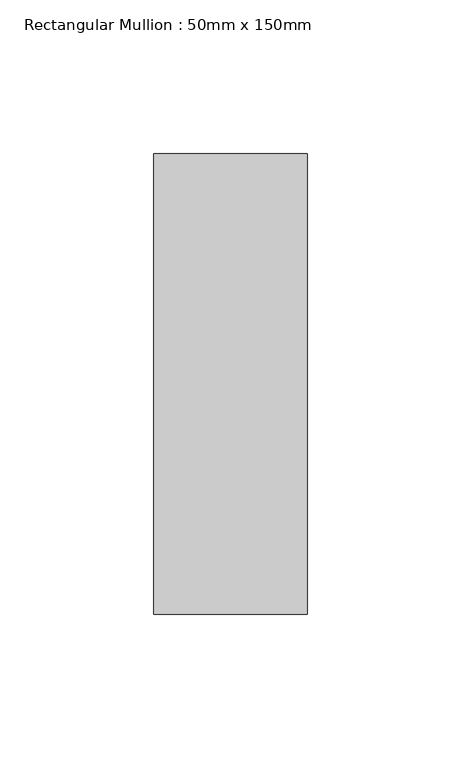
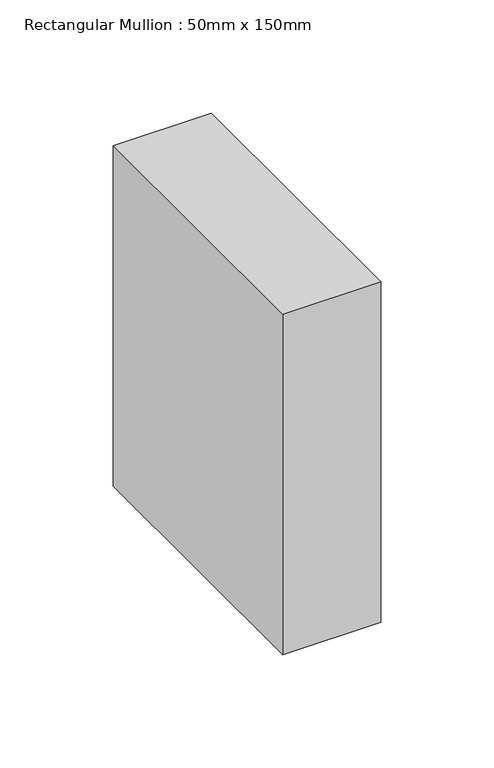
"""IFC4 building model written with IfcOpenShell, lengths in millimetres: member geometry, Rectangular Mullion : 50mm x 150mm."""

from ifc_helpers import new_model, si_unit, frame, origin, place, context, project, spatial, polyline, outline, extrude, source, transform, mapped, element, save


def rectangular_mullion_50mm_x_150mm_93dcffb7(model_context):
    return source(origin(), model_context, "Body", "SweptSolid", [
        extrude(outline(polyline([(0.0, 75.0), (0.0, -75.0), (-50.0, -75.0), (-50.0, 75.0), (0.0, 75.0)])), frame((0.0, 0.0, -183.8383838), z_axis=(0.0, 0.0, 1.0), x_axis=(1.0, 0.0, 0.0)), (0.0, 0.0, 1.0), 183.8383838),
    ])


if __name__ == "__main__":
    model = new_model("IFC4")
    model_context = context("Model", 3, world=origin())
    ifc_project = project(units=[si_unit("LENGTHUNIT", "METRE", prefix="MILLI")], contexts=[model_context])
    site = spatial("IfcSite", under=ifc_project)
    building = spatial("IfcBuilding", under=site)
    placement = place(None, origin())
    rectangular_mullion_50mm_x_150mm_shape = rectangular_mullion_50mm_x_150mm_93dcffb7(model_context)
    element("IfcMember", 1, ObjectType="Rectangular Mullion : 50mm x 150mm", at=placement, inside=building, context=model_context, shape_type="MappedRepresentation", body=[
        mapped(rectangular_mullion_50mm_x_150mm_shape, transform((0.0, 0.0, 0.0), x_axis=(1.0, 0.0, 0.0), y_axis=(0.0, 1.0, 0.0), z_axis=(0.0, 0.0, 1.0))),
    ])
    save(model, "model.ifc")

# Revit data of these elements
# Type "Rectangular Mullion : 50mm x 150mm"
#   built-in parameter 1007304 = 0.492126 (stored number, unit not read)
#   built-in parameter 1007301 = 0.082021 (stored number, unit not read)
#   built-in parameter 1007300 = 0.082021 (stored number, unit not read)
# Element 1 (IfcMember, "Rectangular Mullion : 50mm x 150mm")
#   Materials on its faces: "Aluminum"
# Materials
#   "Aluminum": class "Metal", colour RGB 244 244 244, transparency 0, Description = "Aluminum 6061", Cost = 0
